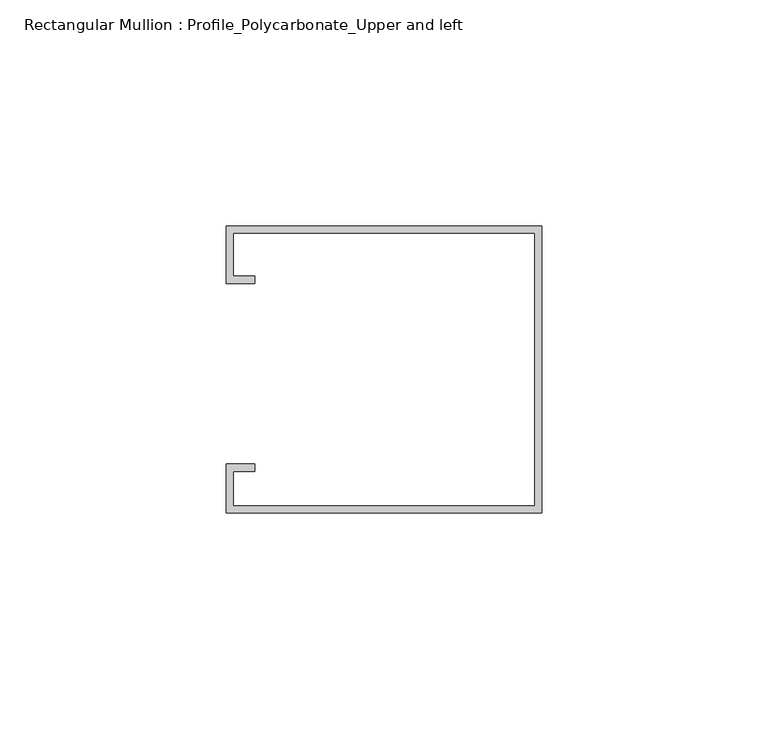
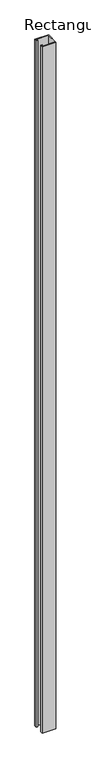
"""IFC4 building model written with IfcOpenShell, lengths in millimetres: member geometry, Rectangular Mullion : Profile_Polycarbonate_Upper and left."""

from ifc_helpers import new_model, si_unit, frame, origin, place, context, project, spatial, polyline, outline, extrude, source, transform, mapped, element, save


def rectangular_mullion_profile_polycarbonate_upper_and_left_bd0ee053(model_context):
    return source(origin(), model_context, "Body", "SweptSolid", [
        extrude(outline(polyline([(0.0, 32.7), (0.0, -30.8), (-69.85, -30.8), (-69.85, -20.0), (-63.5, -20.0), (-63.5, -21.5875), (-68.2625, -21.5875), (-68.2625, -29.2125), (-1.5875, -29.2125), (-1.5875, 31.1125), (-68.2625, 31.1125), (-68.2625, 21.5875), (-63.5, 21.5875), (-63.5, 20.0), (-69.85, 20.0), (-69.85, 32.7), (0.0, 32.7)])), frame((0.0, 0.0, -3697.323634), z_axis=(0.0, 0.0, 1.0), x_axis=(1.0, 0.0, 0.0)), (0.0, 0.0, 1.0), 3697.323634),
    ])


if __name__ == "__main__":
    model = new_model("IFC4")
    model_context = context("Model", 3, world=origin())
    ifc_project = project(units=[si_unit("LENGTHUNIT", "METRE", prefix="MILLI")], contexts=[model_context])
    site = spatial("IfcSite", under=ifc_project)
    building = spatial("IfcBuilding", under=site)
    placement = place(None, origin())
    rectangular_mullion_profile_polycarbonate_upper_and_left_shape = rectangular_mullion_profile_polycarbonate_upper_and_left_bd0ee053(model_context)
    element("IfcMember", 1, ObjectType="Rectangular Mullion : Profile_Polycarbonate_Upper and left", at=placement, inside=building, context=model_context, shape_type="MappedRepresentation", body=[
        mapped(rectangular_mullion_profile_polycarbonate_upper_and_left_shape, transform((0.0, 0.0, 0.0), x_axis=(1.0, 0.0, 0.0), y_axis=(0.0, 1.0, 0.0), z_axis=(0.0, 0.0, 1.0))),
    ])
    save(model, "model.ifc")

# Revit data of these elements
# Type "Rectangular Mullion : Profile_Polycarbonate_Upper and left"
#   built-in parameter 1007322 = 0.208333 (stored number, unit not read)
#   built-in parameter 1007321 = 0.00520833 (stored number, unit not read)
#   built-in parameter 1007320 = 0 (stored number, unit not read)
